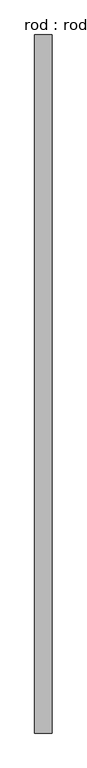
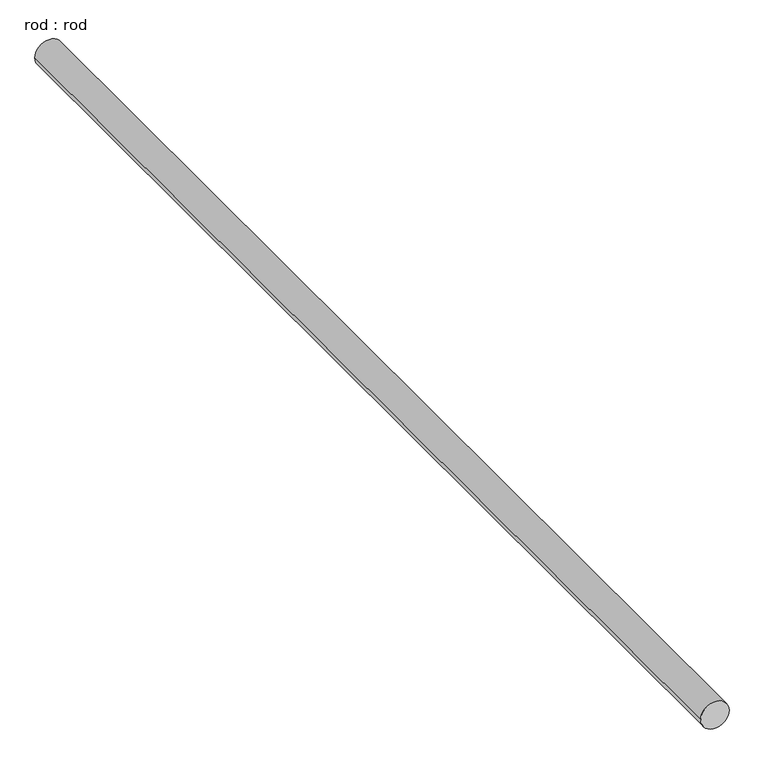
"""IFC4 building model written with IfcOpenShell, lengths in millimetres: proxy geometry, rod : rod."""

import ifcopenshell
import ifcopenshell.guid

model = None  # the IFC model being written
_history = None  # IfcOwnerHistory: only IFC2X3 demands one
_inside = {}  # id of a spatial element -> (the spatial element, [elements in it])
_under = {}  # id of a project, library or spatial element -> (it, [spatial elements below it])
_declared = {}  # id of a project -> (the project, [libraries it declares])
_typed = {}  # id of a type object -> (the type object, [elements of that type])
_made_of = {}  # id of a material, layer set ... -> (it, [elements and type objects made of it])


def new_model(schema):
    """Start an empty IFC model of exactly this schema.

    Asked for "IFC4X3", IfcOpenShell would pick the latest addendum, in which some entities
    have other attributes; the version numbers below select the first issue.
    IFC2X3 requires an IfcOwnerHistory on every rooted entity: one is made here for all.
    """
    global model, _history
    if schema == "IFC4X3":
        model = ifcopenshell.file(schema_version=(4, 3, 0, 0))
    else:
        model = ifcopenshell.file(schema=schema)
    _inside.clear()
    _under.clear()
    _declared.clear()
    _typed.clear()
    _made_of.clear()
    _history = None
    if model.schema == "IFC2X3":
        org = make("IfcOrganization", Name="unknown")
        user = make(
            "IfcPersonAndOrganization",
            ThePerson=make("IfcPerson", FamilyName="unknown"),
            TheOrganization=org,
        )
        app = make(
            "IfcApplication",
            ApplicationDeveloper=org,
            Version="unknown",
            ApplicationFullName="unknown",
            ApplicationIdentifier="unknown",
        )
        _history = make(
            "IfcOwnerHistory",
            OwningUser=user,
            OwningApplication=app,
            ChangeAction="ADDED",
            CreationDate=0,
        )
    return model


def make(cls, **values):
    """One entity of the class cls with the attributes given. An attribute that is None is left unset."""
    return model.create_entity(
        cls, **{name: value for name, value in values.items() if value is not None}
    )


def rooted(cls, **values):
    """An entity with a GlobalId (a new one), such as an element, a storey or a relation."""
    return make(cls, GlobalId=ifcopenshell.guid.new(), OwnerHistory=_history, **values)


def si_unit(unit_type, name, prefix=None):
    """IfcSIUnit, for example si_unit("LENGTHUNIT", "METRE", prefix="MILLI")."""
    return make("IfcSIUnit", UnitType=unit_type, Prefix=prefix, Name=name)


def assignment(units):
    """IfcUnitAssignment: the units of a project."""
    return None if units is None else make("IfcUnitAssignment", Units=units)


def point(xyz):
    """IfcCartesianPoint."""
    return None if xyz is None else make("IfcCartesianPoint", Coordinates=xyz)


def direction(xyz):
    """IfcDirection."""
    return None if xyz is None else make("IfcDirection", DirectionRatios=xyz)


def frame(location, z_axis=None, x_axis=None):
    """IfcAxis2Placement3D, a coordinate frame: its origin and axes. An axis left out is left unset."""
    return make(
        "IfcAxis2Placement3D",
        Location=point(location),
        Axis=direction(z_axis),
        RefDirection=direction(x_axis),
    )


def frame_2d(location, x_axis=None):
    """IfcAxis2Placement2D, a coordinate frame in the plane: its origin and x axis."""
    return make(
        "IfcAxis2Placement2D", Location=point(location), RefDirection=direction(x_axis)
    )


def origin():
    """The frame at (0, 0, 0) with its axes left unset."""
    return frame((0.0, 0.0, 0.0))


def place(relative_to, where):
    """IfcLocalPlacement: puts the frame where relative to a parent placement (None: the world)."""
    return make(
        "IfcLocalPlacement", PlacementRelTo=relative_to, RelativePlacement=where
    )


def context(
    kind, dimensions, precision=None, world=None, true_north=None, identifier=None
):
    """IfcGeometricRepresentationContext, for example the 3D "Model" context."""
    return make(
        "IfcGeometricRepresentationContext",
        ContextIdentifier=identifier,
        ContextType=kind,
        CoordinateSpaceDimension=dimensions,
        Precision=precision,
        WorldCoordinateSystem=world,
        TrueNorth=true_north,
    )


def project(units=None, contexts=None):
    """IfcProject with its units and contexts."""
    return rooted(
        "IfcProject",
        Name="project",
        RepresentationContexts=contexts,
        UnitsInContext=assignment(units),
    )


def spatial(cls, under=None, at=None, **own):
    """A site, building, storey or space (cls), placed at a placement, below another one or the project."""
    s = rooted(cls, ObjectPlacement=at, **own)
    if under is not None:
        _under.setdefault(under.id(), (under, []))[1].append(s)
    return s


def circle_curve(where, radius):
    """IfcCircle in the frame where."""
    return make("IfcCircle", Position=where, Radius=radius)


def trimmed(basis, trim1, trim2, sense, master):
    """IfcTrimmedCurve: the piece of a basis curve between two trims."""
    return make(
        "IfcTrimmedCurve",
        BasisCurve=basis,
        Trim1=trim1,
        Trim2=trim2,
        SenseAgreement=sense,
        MasterRepresentation=master,
    )


def segment(curve, same_sense, transition):
    """IfcCompositeCurveSegment."""
    return make(
        "IfcCompositeCurveSegment",
        Transition=transition,
        SameSense=same_sense,
        ParentCurve=curve,
    )


def composite_curve(segments, self_intersect=None):
    """IfcCompositeCurve: segments joined end to end."""
    return make("IfcCompositeCurve", Segments=segments, SelfIntersect=self_intersect)


def outline(outer, holes=None, kind="AREA"):
    """IfcArbitraryClosedProfileDef: a profile drawn as a closed curve; with holes, ...WithVoids."""
    if holes is None:
        return make("IfcArbitraryClosedProfileDef", ProfileType=kind, OuterCurve=outer)
    return make(
        "IfcArbitraryProfileDefWithVoids",
        ProfileType=kind,
        OuterCurve=outer,
        InnerCurves=holes,
    )


def extrude(swept, where, along, depth):
    """IfcExtrudedAreaSolid: the profile swept, set in the frame where, extruded along a direction by depth."""
    return make(
        "IfcExtrudedAreaSolid",
        SweptArea=swept,
        Position=where,
        ExtrudedDirection=direction(along),
        Depth=depth,
    )


def shape(context_of_items, identifier, shape_type, items):
    """IfcShapeRepresentation: the items that make up one representation, for example the "Body"."""
    return make(
        "IfcShapeRepresentation",
        ContextOfItems=context_of_items,
        RepresentationIdentifier=identifier,
        RepresentationType=shape_type,
        Items=items,
    )


def source(mapping_origin, context_of_items, identifier, shape_type, items):
    """IfcRepresentationMap: a shape defined once, which mapped items show again and again."""
    return make(
        "IfcRepresentationMap",
        MappingOrigin=mapping_origin,
        MappedRepresentation=shape(context_of_items, identifier, shape_type, items),
    )


def transform(
    local_origin,
    x_axis=None,
    y_axis=None,
    z_axis=None,
    scale=None,
    scale2=None,
    scale3=None,
    uniform=True,
):
    """IfcCartesianTransformationOperator3D, or its non-uniform kind. x_axis, y_axis, z_axis: its Axis1, 2, 3."""
    if uniform:
        return make(
            "IfcCartesianTransformationOperator3D",
            Axis1=direction(x_axis),
            Axis2=direction(y_axis),
            LocalOrigin=point(local_origin),
            Scale=scale,
            Axis3=direction(z_axis),
        )
    return make(
        "IfcCartesianTransformationOperator3DnonUniform",
        Axis1=direction(x_axis),
        Axis2=direction(y_axis),
        LocalOrigin=point(local_origin),
        Scale=scale,
        Axis3=direction(z_axis),
        Scale2=scale2,
        Scale3=scale3,
    )


def mapped(mapping_source, mapping_target):
    """IfcMappedItem: shows the shape of a source again, moved by a transform."""
    return make(
        "IfcMappedItem", MappingSource=mapping_source, MappingTarget=mapping_target
    )


def made_of(thing, what):
    """Note that an element or type object is made of a material, layer set ...; save() writes the relation."""
    if what is not None:
        _made_of.setdefault(what.id(), (what, []))[1].append(thing)
    return thing


def element(
    cls,
    number,
    at=None,
    inside=None,
    cuts=None,
    type_object=None,
    material=None,
    context=None,
    identifier="Body",
    shape_type=None,
    held_by="IfcProductDefinitionShape",
    body=None,
    shapes=None,
    **own,
):
    """One element of the class cls, such as IfcWall. Its Tag is "e" and its number.

    at: its placement. inside: the storey or other place that contains it. cuts: it is an
    opening in that element (IfcRelVoidsElement). A single representation is given by context,
    identifier, shape_type and body (its items); several are given by shapes. held_by: the class
    of the entity that holds the representations. save() writes the other relations.
    """
    e = rooted(cls, Tag="e%d" % number, ObjectPlacement=at, **own)
    if body is not None:
        shapes = [shape(context, identifier, shape_type, body)]
    if shapes is not None:
        e.Representation = make(held_by, Representations=shapes)
    if inside is not None:
        _inside.setdefault(inside.id(), (inside, []))[1].append(e)
    if cuts is not None:
        rooted(
            "IfcRelVoidsElement", RelatingBuildingElement=cuts, RelatedOpeningElement=e
        )
    if type_object is not None:
        _typed.setdefault(type_object.id(), (type_object, []))[1].append(e)
    return made_of(e, material)


def aggregate(whole, parts):
    """IfcRelAggregates: a whole, such as a stair, and the parts it consists of."""
    return rooted("IfcRelAggregates", RelatingObject=whole, RelatedObjects=parts)


def save(model, path):
    """Write the relations noted so far, then the file.

    IfcRelAggregates (storeys below a building ...), IfcRelContainedInSpatialStructure (elements
    in a storey), IfcRelDefinesByType, IfcRelAssociatesMaterial and IfcRelDeclares: one each for
    every whole, place, type object, material and project.
    """
    for whole, parts in _under.values():
        aggregate(whole, parts)
    for where, things in _inside.values():
        rooted(
            "IfcRelContainedInSpatialStructure",
            RelatedElements=things,
            RelatingStructure=where,
        )
    for kind, things in _typed.values():
        rooted("IfcRelDefinesByType", RelatedObjects=things, RelatingType=kind)
    for what, things in _made_of.values():
        rooted("IfcRelAssociatesMaterial", RelatedObjects=things, RelatingMaterial=what)
    for by, libraries in _declared.values():
        rooted("IfcRelDeclares", RelatingContext=by, RelatedDefinitions=libraries)
    model.write(path)


def rod_rod_6b01d2ed(model_context):
    return source(origin(), model_context, "Body", "SweptSolid", [
        extrude(outline(composite_curve([segment(trimmed(circle_curve(frame_2d((0.0108462, 0.0)), 200.0), [point((0.0108462, 200.0))], [point((0.0108462, -200.0))], False, "CARTESIAN"), True, "CONTINUOUS"), segment(trimmed(circle_curve(frame_2d((0.0108462, 0.0)), 200.0), [point((0.0108462, -200.0))], [point((0.0108462, 200.0))], False, "CARTESIAN"), True, "CONTINUOUS")], self_intersect=False)), frame((0.0, -4032.2713847, 0.0), z_axis=(0.0, 1.0, 0.0), x_axis=(0.0, 0.0, 1.0)), (0.0, 0.0, 1.0), 16250.0),
    ])


if __name__ == "__main__":
    model = new_model("IFC4")
    model_context = context("Model", 3, world=origin())
    ifc_project = project(units=[si_unit("LENGTHUNIT", "METRE", prefix="MILLI")], contexts=[model_context])
    site = spatial("IfcSite", under=ifc_project)
    building = spatial("IfcBuilding", under=site)
    placement = place(None, origin())
    rod_rod_shape = rod_rod_6b01d2ed(model_context)
    element("IfcBuildingElementProxy", 1, Name="rod : rod", ObjectType="rod : rod", at=placement, inside=building, context=model_context, shape_type="MappedRepresentation", body=[
        mapped(rod_rod_shape, transform((0.0, 0.0, 0.0), x_axis=(1.0, 0.0, 0.0), y_axis=(0.0, 1.0, 0.0), z_axis=(0.0, 0.0, 1.0))),
    ])
    save(model, "model.ifc")

# Revit data of these elements
# Type "rod : rod"
#   Default Elevation = 0
